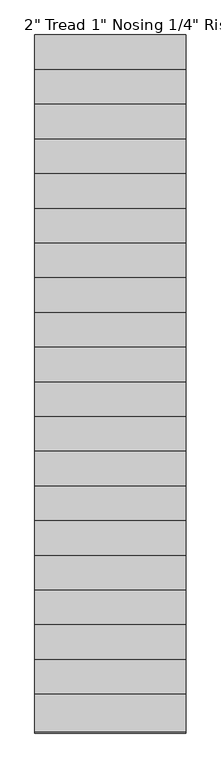
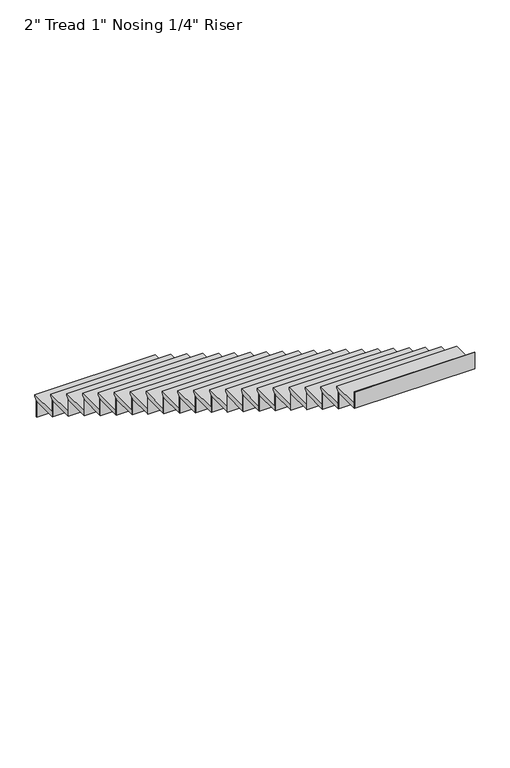
"""IFC4 building model written with IfcOpenShell, lengths in millimetres: stair flight geometry."""

import ifcopenshell
import ifcopenshell.guid

model = None  # the IFC model being written
_history = None  # IfcOwnerHistory: only IFC2X3 demands one
_inside = {}  # id of a spatial element -> (the spatial element, [elements in it])
_under = {}  # id of a project, library or spatial element -> (it, [spatial elements below it])
_declared = {}  # id of a project -> (the project, [libraries it declares])
_typed = {}  # id of a type object -> (the type object, [elements of that type])
_made_of = {}  # id of a material, layer set ... -> (it, [elements and type objects made of it])


def new_model(schema):
    """Start an empty IFC model of exactly this schema.

    Asked for "IFC4X3", IfcOpenShell would pick the latest addendum, in which some entities
    have other attributes; the version numbers below select the first issue.
    IFC2X3 requires an IfcOwnerHistory on every rooted entity: one is made here for all.
    """
    global model, _history
    if schema == "IFC4X3":
        model = ifcopenshell.file(schema_version=(4, 3, 0, 0))
    else:
        model = ifcopenshell.file(schema=schema)
    _inside.clear()
    _under.clear()
    _declared.clear()
    _typed.clear()
    _made_of.clear()
    _history = None
    if model.schema == "IFC2X3":
        org = make("IfcOrganization", Name="unknown")
        user = make(
            "IfcPersonAndOrganization",
            ThePerson=make("IfcPerson", FamilyName="unknown"),
            TheOrganization=org,
        )
        app = make(
            "IfcApplication",
            ApplicationDeveloper=org,
            Version="unknown",
            ApplicationFullName="unknown",
            ApplicationIdentifier="unknown",
        )
        _history = make(
            "IfcOwnerHistory",
            OwningUser=user,
            OwningApplication=app,
            ChangeAction="ADDED",
            CreationDate=0,
        )
    return model


def make(cls, **values):
    """One entity of the class cls with the attributes given. An attribute that is None is left unset."""
    return model.create_entity(
        cls, **{name: value for name, value in values.items() if value is not None}
    )


def rooted(cls, **values):
    """An entity with a GlobalId (a new one), such as an element, a storey or a relation."""
    return make(cls, GlobalId=ifcopenshell.guid.new(), OwnerHistory=_history, **values)


def si_unit(unit_type, name, prefix=None):
    """IfcSIUnit, for example si_unit("LENGTHUNIT", "METRE", prefix="MILLI")."""
    return make("IfcSIUnit", UnitType=unit_type, Prefix=prefix, Name=name)


def assignment(units):
    """IfcUnitAssignment: the units of a project."""
    return None if units is None else make("IfcUnitAssignment", Units=units)


def point(xyz):
    """IfcCartesianPoint."""
    return None if xyz is None else make("IfcCartesianPoint", Coordinates=xyz)


def direction(xyz):
    """IfcDirection."""
    return None if xyz is None else make("IfcDirection", DirectionRatios=xyz)


def frame(location, z_axis=None, x_axis=None):
    """IfcAxis2Placement3D, a coordinate frame: its origin and axes. An axis left out is left unset."""
    return make(
        "IfcAxis2Placement3D",
        Location=point(location),
        Axis=direction(z_axis),
        RefDirection=direction(x_axis),
    )


def origin():
    """The frame at (0, 0, 0) with its axes left unset."""
    return frame((0.0, 0.0, 0.0))


def place(relative_to, where):
    """IfcLocalPlacement: puts the frame where relative to a parent placement (None: the world)."""
    return make(
        "IfcLocalPlacement", PlacementRelTo=relative_to, RelativePlacement=where
    )


def context(
    kind, dimensions, precision=None, world=None, true_north=None, identifier=None
):
    """IfcGeometricRepresentationContext, for example the 3D "Model" context."""
    return make(
        "IfcGeometricRepresentationContext",
        ContextIdentifier=identifier,
        ContextType=kind,
        CoordinateSpaceDimension=dimensions,
        Precision=precision,
        WorldCoordinateSystem=world,
        TrueNorth=true_north,
    )


def project(units=None, contexts=None):
    """IfcProject with its units and contexts."""
    return rooted(
        "IfcProject",
        Name="project",
        RepresentationContexts=contexts,
        UnitsInContext=assignment(units),
    )


def spatial(cls, under=None, at=None, **own):
    """A site, building, storey or space (cls), placed at a placement, below another one or the project."""
    s = rooted(cls, ObjectPlacement=at, **own)
    if under is not None:
        _under.setdefault(under.id(), (under, []))[1].append(s)
    return s


def polyline(points):
    """IfcPolyline through the points."""
    return make("IfcPolyline", Points=[point(p) for p in points])


def outline(outer, holes=None, kind="AREA"):
    """IfcArbitraryClosedProfileDef: a profile drawn as a closed curve; with holes, ...WithVoids."""
    if holes is None:
        return make("IfcArbitraryClosedProfileDef", ProfileType=kind, OuterCurve=outer)
    return make(
        "IfcArbitraryProfileDefWithVoids",
        ProfileType=kind,
        OuterCurve=outer,
        InnerCurves=holes,
    )


def extrude(swept, where, along, depth):
    """IfcExtrudedAreaSolid: the profile swept, set in the frame where, extruded along a direction by depth."""
    return make(
        "IfcExtrudedAreaSolid",
        SweptArea=swept,
        Position=where,
        ExtrudedDirection=direction(along),
        Depth=depth,
    )


def shape(context_of_items, identifier, shape_type, items):
    """IfcShapeRepresentation: the items that make up one representation, for example the "Body"."""
    return make(
        "IfcShapeRepresentation",
        ContextOfItems=context_of_items,
        RepresentationIdentifier=identifier,
        RepresentationType=shape_type,
        Items=items,
    )


def source(mapping_origin, context_of_items, identifier, shape_type, items):
    """IfcRepresentationMap: a shape defined once, which mapped items show again and again."""
    return make(
        "IfcRepresentationMap",
        MappingOrigin=mapping_origin,
        MappedRepresentation=shape(context_of_items, identifier, shape_type, items),
    )


def transform(
    local_origin,
    x_axis=None,
    y_axis=None,
    z_axis=None,
    scale=None,
    scale2=None,
    scale3=None,
    uniform=True,
):
    """IfcCartesianTransformationOperator3D, or its non-uniform kind. x_axis, y_axis, z_axis: its Axis1, 2, 3."""
    if uniform:
        return make(
            "IfcCartesianTransformationOperator3D",
            Axis1=direction(x_axis),
            Axis2=direction(y_axis),
            LocalOrigin=point(local_origin),
            Scale=scale,
            Axis3=direction(z_axis),
        )
    return make(
        "IfcCartesianTransformationOperator3DnonUniform",
        Axis1=direction(x_axis),
        Axis2=direction(y_axis),
        LocalOrigin=point(local_origin),
        Scale=scale,
        Axis3=direction(z_axis),
        Scale2=scale2,
        Scale3=scale3,
    )


def mapped(mapping_source, mapping_target):
    """IfcMappedItem: shows the shape of a source again, moved by a transform."""
    return make(
        "IfcMappedItem", MappingSource=mapping_source, MappingTarget=mapping_target
    )


def made_of(thing, what):
    """Note that an element or type object is made of a material, layer set ...; save() writes the relation."""
    if what is not None:
        _made_of.setdefault(what.id(), (what, []))[1].append(thing)
    return thing


def element(
    cls,
    number,
    at=None,
    inside=None,
    cuts=None,
    type_object=None,
    material=None,
    context=None,
    identifier="Body",
    shape_type=None,
    held_by="IfcProductDefinitionShape",
    body=None,
    shapes=None,
    **own,
):
    """One element of the class cls, such as IfcWall. Its Tag is "e" and its number.

    at: its placement. inside: the storey or other place that contains it. cuts: it is an
    opening in that element (IfcRelVoidsElement). A single representation is given by context,
    identifier, shape_type and body (its items); several are given by shapes. held_by: the class
    of the entity that holds the representations. save() writes the other relations.
    """
    e = rooted(cls, Tag="e%d" % number, ObjectPlacement=at, **own)
    if body is not None:
        shapes = [shape(context, identifier, shape_type, body)]
    if shapes is not None:
        e.Representation = make(held_by, Representations=shapes)
    if inside is not None:
        _inside.setdefault(inside.id(), (inside, []))[1].append(e)
    if cuts is not None:
        rooted(
            "IfcRelVoidsElement", RelatingBuildingElement=cuts, RelatedOpeningElement=e
        )
    if type_object is not None:
        _typed.setdefault(type_object.id(), (type_object, []))[1].append(e)
    return made_of(e, material)


def aggregate(whole, parts):
    """IfcRelAggregates: a whole, such as a stair, and the parts it consists of."""
    return rooted("IfcRelAggregates", RelatingObject=whole, RelatedObjects=parts)


def save(model, path):
    """Write the relations noted so far, then the file.

    IfcRelAggregates (storeys below a building ...), IfcRelContainedInSpatialStructure (elements
    in a storey), IfcRelDefinesByType, IfcRelAssociatesMaterial and IfcRelDeclares: one each for
    every whole, place, type object, material and project.
    """
    for whole, parts in _under.values():
        aggregate(whole, parts)
    for where, things in _inside.values():
        rooted(
            "IfcRelContainedInSpatialStructure",
            RelatedElements=things,
            RelatingStructure=where,
        )
    for kind, things in _typed.values():
        rooted("IfcRelDefinesByType", RelatedObjects=things, RelatingType=kind)
    for what, things in _made_of.values():
        rooted("IfcRelAssociatesMaterial", RelatedObjects=things, RelatingMaterial=what)
    for by, libraries in _declared.values():
        rooted("IfcRelDeclares", RelatingContext=by, RelatedDefinitions=libraries)
    model.write(path)


def stair_flight_5309da95(model_context):
    return source(origin(), model_context, "Body", "SweptSolid", [
        extrude(outline(polyline([(-5103.3507921, 1393.3714286), (-4798.5507921, 1393.3714286), (-4798.5507921, 1374.3214286), (-4823.9507921, 1348.9214286), (-4823.9507921, 1342.5714286), (-5103.3507921, 1342.5714286), (-5103.3507921, 1393.3714286)])), frame((2890.4601743, 0.0, 0.0), z_axis=(1.0, 0.0, 0.0), x_axis=(0.0, 1.0, 0.0)), (0.0, 0.0, 1.0), 1219.2),
        extrude(outline(polyline([(2890.4601743, -4830.3007921), (2890.4601743, -4823.9507921), (4109.6601743, -4823.9507921), (4109.6601743, -4830.3007921), (2890.4601743, -4830.3007921)])), frame((0.0, 0.0, 1168.4), z_axis=(0.0, 0.0, 1.0), x_axis=(1.0, 0.0, 0.0)), (0.0, 0.0, 1.0), 174.1714286),
        extrude(outline(polyline([(2890.4601743, -5109.7007921), (2890.4601743, -5103.3507921), (4109.6601743, -5103.3507921), (4109.6601743, -5109.7007921), (2890.4601743, -5109.7007921)])), frame((0.0, 0.0, 1342.5714286), z_axis=(0.0, 0.0, 1.0), x_axis=(1.0, 0.0, 0.0)), (0.0, 0.0, 1.0), 174.1714286),
        extrude(outline(polyline([(-5382.7507921, 1567.5428571), (-5077.9507921, 1567.5428571), (-5077.9507921, 1548.4928571), (-5103.3507921, 1523.0928571), (-5103.3507921, 1516.7428571), (-5382.7507921, 1516.7428571), (-5382.7507921, 1567.5428571)])), frame((2890.4601743, 0.0, 0.0), z_axis=(1.0, 0.0, 0.0), x_axis=(0.0, 1.0, 0.0)), (0.0, 0.0, 1.0), 1219.2),
        extrude(outline(polyline([(2890.4601743, -5389.1007921), (2890.4601743, -5382.7507921), (4109.6601743, -5382.7507921), (4109.6601743, -5389.1007921), (2890.4601743, -5389.1007921)])), frame((0.0, 0.0, 1516.7428571), z_axis=(0.0, 0.0, 1.0), x_axis=(1.0, 0.0, 0.0)), (0.0, 0.0, 1.0), 174.1714286),
        extrude(outline(polyline([(-5662.1507921, 1741.7142857), (-5357.3507921, 1741.7142857), (-5357.3507921, 1722.6642857), (-5382.7507921, 1697.2642857), (-5382.7507921, 1690.9142857), (-5662.1507921, 1690.9142857), (-5662.1507921, 1741.7142857)])), frame((2890.4601743, 0.0, 0.0), z_axis=(1.0, 0.0, 0.0), x_axis=(0.0, 1.0, 0.0)), (0.0, 0.0, 1.0), 1219.2),
        extrude(outline(polyline([(2890.4601743, -5668.5007921), (2890.4601743, -5662.1507921), (4109.6601743, -5662.1507921), (4109.6601743, -5668.5007921), (2890.4601743, -5668.5007921)])), frame((0.0, 0.0, 1690.9142857), z_axis=(0.0, 0.0, 1.0), x_axis=(1.0, 0.0, 0.0)), (0.0, 0.0, 1.0), 174.1714286),
        extrude(outline(polyline([(-5941.5507921, 1915.8857143), (-5636.7507921, 1915.8857143), (-5636.7507921, 1896.8357143), (-5662.1507921, 1871.4357143), (-5662.1507921, 1865.0857143), (-5941.5507921, 1865.0857143), (-5941.5507921, 1915.8857143)])), frame((2890.4601743, 0.0, 0.0), z_axis=(1.0, 0.0, 0.0), x_axis=(0.0, 1.0, 0.0)), (0.0, 0.0, 1.0), 1219.2),
        extrude(outline(polyline([(2890.4601743, -5947.9007921), (2890.4601743, -5941.5507921), (4109.6601743, -5941.5507921), (4109.6601743, -5947.9007921), (2890.4601743, -5947.9007921)])), frame((0.0, 0.0, 1865.0857143), z_axis=(0.0, 0.0, 1.0), x_axis=(1.0, 0.0, 0.0)), (0.0, 0.0, 1.0), 174.1714286),
        extrude(outline(polyline([(-6220.9507921, 2090.0571429), (-5916.1507921, 2090.0571429), (-5916.1507921, 2071.0071429), (-5941.5507921, 2045.6071429), (-5941.5507921, 2039.2571429), (-6220.9507921, 2039.2571429), (-6220.9507921, 2090.0571429)])), frame((2890.4601743, 0.0, 0.0), z_axis=(1.0, 0.0, 0.0), x_axis=(0.0, 1.0, 0.0)), (0.0, 0.0, 1.0), 1219.2),
        extrude(outline(polyline([(2890.4601743, -6227.3007921), (2890.4601743, -6220.9507921), (4109.6601743, -6220.9507921), (4109.6601743, -6227.3007921), (2890.4601743, -6227.3007921)])), frame((0.0, 0.0, 2039.2571429), z_axis=(0.0, 0.0, 1.0), x_axis=(1.0, 0.0, 0.0)), (0.0, 0.0, 1.0), 174.1714286),
        extrude(outline(polyline([(-6500.3507921, 2264.2285714), (-6195.5507921, 2264.2285714), (-6195.5507921, 2245.1785714), (-6220.9507921, 2219.7785714), (-6220.9507921, 2213.4285714), (-6500.3507921, 2213.4285714), (-6500.3507921, 2264.2285714)])), frame((2890.4601743, 0.0, 0.0), z_axis=(1.0, 0.0, 0.0), x_axis=(0.0, 1.0, 0.0)), (0.0, 0.0, 1.0), 1219.2),
        extrude(outline(polyline([(2890.4601743, -6506.7007921), (2890.4601743, -6500.3507921), (4109.6601743, -6500.3507921), (4109.6601743, -6506.7007921), (2890.4601743, -6506.7007921)])), frame((0.0, 0.0, 2213.4285714), z_axis=(0.0, 0.0, 1.0), x_axis=(1.0, 0.0, 0.0)), (0.0, 0.0, 1.0), 174.1714286),
        extrude(outline(polyline([(-6779.7507921, 2438.4), (-6474.9507921, 2438.4), (-6474.9507921, 2419.35), (-6500.3507921, 2393.95), (-6500.3507921, 2387.6), (-6779.7507921, 2387.6), (-6779.7507921, 2438.4)])), frame((2890.4601743, 0.0, 0.0), z_axis=(1.0, 0.0, 0.0), x_axis=(0.0, 1.0, 0.0)), (0.0, 0.0, 1.0), 1219.2),
        extrude(outline(polyline([(2890.4601743, -6786.1007921), (2890.4601743, -6779.7507921), (4109.6601743, -6779.7507921), (4109.6601743, -6786.1007921), (2890.4601743, -6786.1007921)])), frame((0.0, 0.0, 2387.6), z_axis=(0.0, 0.0, 1.0), x_axis=(1.0, 0.0, 0.0)), (0.0, 0.0, 1.0), 174.1714286),
        extrude(outline(polyline([(-7059.1507921, 2612.5714286), (-6754.3507921, 2612.5714286), (-6754.3507921, 2593.5214286), (-6779.7507921, 2568.1214286), (-6779.7507921, 2561.7714286), (-7059.1507921, 2561.7714286), (-7059.1507921, 2612.5714286)])), frame((2890.4601743, 0.0, 0.0), z_axis=(1.0, 0.0, 0.0), x_axis=(0.0, 1.0, 0.0)), (0.0, 0.0, 1.0), 1219.2),
        extrude(outline(polyline([(2890.4601743, -7065.5007921), (2890.4601743, -7059.1507921), (4109.6601743, -7059.1507921), (4109.6601743, -7065.5007921), (2890.4601743, -7065.5007921)])), frame((0.0, 0.0, 2561.7714286), z_axis=(0.0, 0.0, 1.0), x_axis=(1.0, 0.0, 0.0)), (0.0, 0.0, 1.0), 174.1714286),
        extrude(outline(polyline([(-7338.5507921, 2786.7428571), (-7033.7507921, 2786.7428571), (-7033.7507921, 2767.6928571), (-7059.1507921, 2742.2928571), (-7059.1507921, 2735.9428571), (-7338.5507921, 2735.9428571), (-7338.5507921, 2786.7428571)])), frame((2890.4601743, 0.0, 0.0), z_axis=(1.0, 0.0, 0.0), x_axis=(0.0, 1.0, 0.0)), (0.0, 0.0, 1.0), 1219.2),
        extrude(outline(polyline([(2890.4601743, -7344.9007921), (2890.4601743, -7338.5507921), (4109.6601743, -7338.5507921), (4109.6601743, -7344.9007921), (2890.4601743, -7344.9007921)])), frame((0.0, 0.0, 2735.9428571), z_axis=(0.0, 0.0, 1.0), x_axis=(1.0, 0.0, 0.0)), (0.0, 0.0, 1.0), 174.1714286),
        extrude(outline(polyline([(-7617.9507921, 2960.9142857), (-7313.1507921, 2960.9142857), (-7313.1507921, 2941.8642857), (-7338.5507921, 2916.4642857), (-7338.5507921, 2910.1142857), (-7617.9507921, 2910.1142857), (-7617.9507921, 2960.9142857)])), frame((2890.4601743, 0.0, 0.0), z_axis=(1.0, 0.0, 0.0), x_axis=(0.0, 1.0, 0.0)), (0.0, 0.0, 1.0), 1219.2),
        extrude(outline(polyline([(2890.4601743, -7624.3007921), (2890.4601743, -7617.9507921), (4109.6601743, -7617.9507921), (4109.6601743, -7624.3007921), (2890.4601743, -7624.3007921)])), frame((0.0, 0.0, 2910.1142857), z_axis=(0.0, 0.0, 1.0), x_axis=(1.0, 0.0, 0.0)), (0.0, 0.0, 1.0), 174.1714286),
        extrude(outline(polyline([(-7897.3507921, 3135.0857143), (-7592.5507921, 3135.0857143), (-7592.5507921, 3116.0357143), (-7617.9507921, 3090.6357143), (-7617.9507921, 3084.2857143), (-7897.3507921, 3084.2857143), (-7897.3507921, 3135.0857143)])), frame((2890.4601743, 0.0, 0.0), z_axis=(1.0, 0.0, 0.0), x_axis=(0.0, 1.0, 0.0)), (0.0, 0.0, 1.0), 1219.2),
        extrude(outline(polyline([(2890.4601743, -7903.7007921), (2890.4601743, -7897.3507921), (4109.6601743, -7897.3507921), (4109.6601743, -7903.7007921), (2890.4601743, -7903.7007921)])), frame((0.0, 0.0, 3084.2857143), z_axis=(0.0, 0.0, 1.0), x_axis=(1.0, 0.0, 0.0)), (0.0, 0.0, 1.0), 174.1714286),
        extrude(outline(polyline([(-8176.7507921, 3309.2571429), (-7871.9507921, 3309.2571429), (-7871.9507921, 3290.2071429), (-7897.3507921, 3264.8071429), (-7897.3507921, 3258.4571429), (-8176.7507921, 3258.4571429), (-8176.7507921, 3309.2571429)])), frame((2890.4601743, 0.0, 0.0), z_axis=(1.0, 0.0, 0.0), x_axis=(0.0, 1.0, 0.0)), (0.0, 0.0, 1.0), 1219.2),
        extrude(outline(polyline([(2890.4601743, -8183.1007921), (2890.4601743, -8176.7507921), (4109.6601743, -8176.7507921), (4109.6601743, -8183.1007921), (2890.4601743, -8183.1007921)])), frame((0.0, 0.0, 3258.4571429), z_axis=(0.0, 0.0, 1.0), x_axis=(1.0, 0.0, 0.0)), (0.0, 0.0, 1.0), 174.1714286),
        extrude(outline(polyline([(-8456.1507921, 3483.4285714), (-8151.3507921, 3483.4285714), (-8151.3507921, 3464.3785714), (-8176.7507921, 3438.9785714), (-8176.7507921, 3432.6285714), (-8456.1507921, 3432.6285714), (-8456.1507921, 3483.4285714)])), frame((2890.4601743, 0.0, 0.0), z_axis=(1.0, 0.0, 0.0), x_axis=(0.0, 1.0, 0.0)), (0.0, 0.0, 1.0), 1219.2),
        extrude(outline(polyline([(2890.4601743, -8462.5007921), (2890.4601743, -8456.1507921), (4109.6601743, -8456.1507921), (4109.6601743, -8462.5007921), (2890.4601743, -8462.5007921)])), frame((0.0, 0.0, 3432.6285714), z_axis=(0.0, 0.0, 1.0), x_axis=(1.0, 0.0, 0.0)), (0.0, 0.0, 1.0), 174.1714286),
        extrude(outline(polyline([(-8735.5507921, 3657.6), (-8430.7507921, 3657.6), (-8430.7507921, 3638.55), (-8456.1507921, 3613.15), (-8456.1507921, 3606.8), (-8735.5507921, 3606.8), (-8735.5507921, 3657.6)])), frame((2890.4601743, 0.0, 0.0), z_axis=(1.0, 0.0, 0.0), x_axis=(0.0, 1.0, 0.0)), (0.0, 0.0, 1.0), 1219.2),
        extrude(outline(polyline([(2890.4601743, -8741.9007921), (2890.4601743, -8735.5507921), (4109.6601743, -8735.5507921), (4109.6601743, -8741.9007921), (2890.4601743, -8741.9007921)])), frame((0.0, 0.0, 3606.8), z_axis=(0.0, 0.0, 1.0), x_axis=(1.0, 0.0, 0.0)), (0.0, 0.0, 1.0), 174.1714286),
        extrude(outline(polyline([(-9014.9507921, 3831.7714286), (-8710.1507921, 3831.7714286), (-8710.1507921, 3812.7214286), (-8735.5507921, 3787.3214286), (-8735.5507921, 3780.9714286), (-9014.9507921, 3780.9714286), (-9014.9507921, 3831.7714286)])), frame((2890.4601743, 0.0, 0.0), z_axis=(1.0, 0.0, 0.0), x_axis=(0.0, 1.0, 0.0)), (0.0, 0.0, 1.0), 1219.2),
        extrude(outline(polyline([(2890.4601743, -9021.3007921), (2890.4601743, -9014.9507921), (4109.6601743, -9014.9507921), (4109.6601743, -9021.3007921), (2890.4601743, -9021.3007921)])), frame((0.0, 0.0, 3780.9714286), z_axis=(0.0, 0.0, 1.0), x_axis=(1.0, 0.0, 0.0)), (0.0, 0.0, 1.0), 174.1714286),
        extrude(outline(polyline([(-9294.3507921, 4005.9428571), (-8989.5507921, 4005.9428571), (-8989.5507921, 3986.8928571), (-9014.9507921, 3961.4928571), (-9014.9507921, 3955.1428571), (-9294.3507921, 3955.1428571), (-9294.3507921, 4005.9428571)])), frame((2890.4601743, 0.0, 0.0), z_axis=(1.0, 0.0, 0.0), x_axis=(0.0, 1.0, 0.0)), (0.0, 0.0, 1.0), 1219.2),
        extrude(outline(polyline([(2890.4601743, -9300.7007921), (2890.4601743, -9294.3507921), (4109.6601743, -9294.3507921), (4109.6601743, -9300.7007921), (2890.4601743, -9300.7007921)])), frame((0.0, 0.0, 3955.1428571), z_axis=(0.0, 0.0, 1.0), x_axis=(1.0, 0.0, 0.0)), (0.0, 0.0, 1.0), 174.1714286),
        extrude(outline(polyline([(-9573.7507921, 4180.1142857), (-9268.9507921, 4180.1142857), (-9268.9507921, 4161.0642857), (-9294.3507921, 4135.6642857), (-9294.3507921, 4129.3142857), (-9573.7507921, 4129.3142857), (-9573.7507921, 4180.1142857)])), frame((2890.4601743, 0.0, 0.0), z_axis=(1.0, 0.0, 0.0), x_axis=(0.0, 1.0, 0.0)), (0.0, 0.0, 1.0), 1219.2),
        extrude(outline(polyline([(2890.4601743, -9580.1007921), (2890.4601743, -9573.7507921), (4109.6601743, -9573.7507921), (4109.6601743, -9580.1007921), (2890.4601743, -9580.1007921)])), frame((0.0, 0.0, 4129.3142857), z_axis=(0.0, 0.0, 1.0), x_axis=(1.0, 0.0, 0.0)), (0.0, 0.0, 1.0), 174.1714286),
        extrude(outline(polyline([(-9853.1507921, 4354.2857143), (-9548.3507921, 4354.2857143), (-9548.3507921, 4335.2357143), (-9573.7507921, 4309.8357143), (-9573.7507921, 4303.4857143), (-9853.1507921, 4303.4857143), (-9853.1507921, 4354.2857143)])), frame((2890.4601743, 0.0, 0.0), z_axis=(1.0, 0.0, 0.0), x_axis=(0.0, 1.0, 0.0)), (0.0, 0.0, 1.0), 1219.2),
        extrude(outline(polyline([(2890.4601743, -9859.5007921), (2890.4601743, -9853.1507921), (4109.6601743, -9853.1507921), (4109.6601743, -9859.5007921), (2890.4601743, -9859.5007921)])), frame((0.0, 0.0, 4303.4857143), z_axis=(0.0, 0.0, 1.0), x_axis=(1.0, 0.0, 0.0)), (0.0, 0.0, 1.0), 174.1714286),
        extrude(outline(polyline([(-10132.5507921, 4528.4571429), (-9827.7507921, 4528.4571429), (-9827.7507921, 4509.4071429), (-9853.1507921, 4484.0071429), (-9853.1507921, 4477.6571429), (-10132.5507921, 4477.6571429), (-10132.5507921, 4528.4571429)])), frame((2890.4601743, 0.0, 0.0), z_axis=(1.0, 0.0, 0.0), x_axis=(0.0, 1.0, 0.0)), (0.0, 0.0, 1.0), 1219.2),
        extrude(outline(polyline([(2890.4601743, -10138.9007921), (2890.4601743, -10132.5507921), (4109.6601743, -10132.5507921), (4109.6601743, -10138.9007921), (2890.4601743, -10138.9007921)])), frame((0.0, 0.0, 4477.6571429), z_axis=(0.0, 0.0, 1.0), x_axis=(1.0, 0.0, 0.0)), (0.0, 0.0, 1.0), 174.1714286),
        extrude(outline(polyline([(2890.4601743, -10418.3007921), (2890.4601743, -10411.9507921), (4109.6601743, -10411.9507921), (4109.6601743, -10418.3007921), (2890.4601743, -10418.3007921)])), frame((0.0, 0.0, 4651.8285714), z_axis=(0.0, 0.0, 1.0), x_axis=(1.0, 0.0, 0.0)), (0.0, 0.0, 1.0), 174.1714286),
        extrude(outline(polyline([(-10411.9507921, 4702.6285714), (-10107.1507921, 4702.6285714), (-10107.1507921, 4683.5785714), (-10132.5507921, 4658.1785714), (-10132.5507921, 4651.8285714), (-10411.9507921, 4651.8285714), (-10411.9507921, 4702.6285714)])), frame((2890.4601743, 0.0, 0.0), z_axis=(1.0, 0.0, 0.0), x_axis=(0.0, 1.0, 0.0)), (0.0, 0.0, 1.0), 1219.2),
    ])


if __name__ == "__main__":
    model = new_model("IFC4")
    model_context = context("Model", 3, world=origin())
    ifc_project = project(units=[si_unit("LENGTHUNIT", "METRE", prefix="MILLI")], contexts=[model_context])
    site = spatial("IfcSite", under=ifc_project)
    building = spatial("IfcBuilding", under=site)
    placement = place(None, origin())
    stair_flight_shape = stair_flight_5309da95(model_context)
    element("IfcStairFlight", 1, ObjectType="2\" Tread 1\" Nosing 1/4\" Riser", at=placement, inside=building, context=model_context, shape_type="MappedRepresentation", body=[
        mapped(stair_flight_shape, transform((0.0, 0.0, 0.0), x_axis=(1.0, 0.0, 0.0), y_axis=(0.0, 1.0, 0.0), z_axis=(0.0, 0.0, 1.0))),
    ])
    save(model, "model.ifc")
